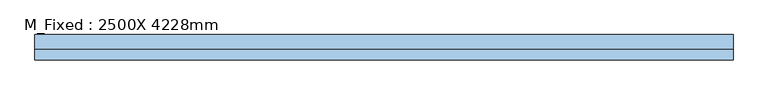
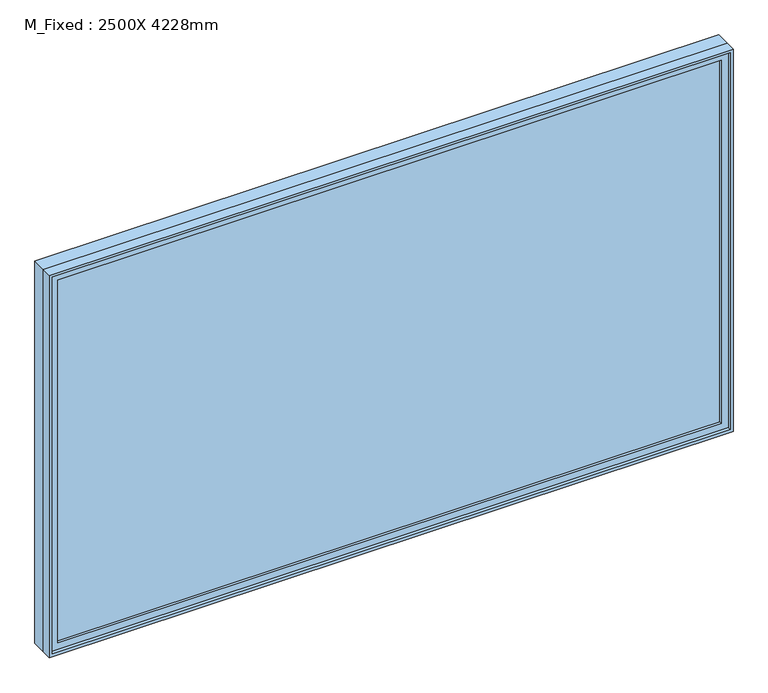
"""IFC4 building model written with IfcOpenShell, lengths in millimetres: window geometry, M_Fixed : 2500X 4228mm."""

import ifcopenshell
import ifcopenshell.guid

model = None  # the IFC model being written
_history = None  # IfcOwnerHistory: only IFC2X3 demands one
_inside = {}  # id of a spatial element -> (the spatial element, [elements in it])
_under = {}  # id of a project, library or spatial element -> (it, [spatial elements below it])
_declared = {}  # id of a project -> (the project, [libraries it declares])
_typed = {}  # id of a type object -> (the type object, [elements of that type])
_made_of = {}  # id of a material, layer set ... -> (it, [elements and type objects made of it])


def new_model(schema):
    """Start an empty IFC model of exactly this schema.

    Asked for "IFC4X3", IfcOpenShell would pick the latest addendum, in which some entities
    have other attributes; the version numbers below select the first issue.
    IFC2X3 requires an IfcOwnerHistory on every rooted entity: one is made here for all.
    """
    global model, _history
    if schema == "IFC4X3":
        model = ifcopenshell.file(schema_version=(4, 3, 0, 0))
    else:
        model = ifcopenshell.file(schema=schema)
    _inside.clear()
    _under.clear()
    _declared.clear()
    _typed.clear()
    _made_of.clear()
    _history = None
    if model.schema == "IFC2X3":
        org = make("IfcOrganization", Name="unknown")
        user = make(
            "IfcPersonAndOrganization",
            ThePerson=make("IfcPerson", FamilyName="unknown"),
            TheOrganization=org,
        )
        app = make(
            "IfcApplication",
            ApplicationDeveloper=org,
            Version="unknown",
            ApplicationFullName="unknown",
            ApplicationIdentifier="unknown",
        )
        _history = make(
            "IfcOwnerHistory",
            OwningUser=user,
            OwningApplication=app,
            ChangeAction="ADDED",
            CreationDate=0,
        )
    return model


def make(cls, **values):
    """One entity of the class cls with the attributes given. An attribute that is None is left unset."""
    return model.create_entity(
        cls, **{name: value for name, value in values.items() if value is not None}
    )


def rooted(cls, **values):
    """An entity with a GlobalId (a new one), such as an element, a storey or a relation."""
    return make(cls, GlobalId=ifcopenshell.guid.new(), OwnerHistory=_history, **values)


def si_unit(unit_type, name, prefix=None):
    """IfcSIUnit, for example si_unit("LENGTHUNIT", "METRE", prefix="MILLI")."""
    return make("IfcSIUnit", UnitType=unit_type, Prefix=prefix, Name=name)


def assignment(units):
    """IfcUnitAssignment: the units of a project."""
    return None if units is None else make("IfcUnitAssignment", Units=units)


def point(xyz):
    """IfcCartesianPoint."""
    return None if xyz is None else make("IfcCartesianPoint", Coordinates=xyz)


def direction(xyz):
    """IfcDirection."""
    return None if xyz is None else make("IfcDirection", DirectionRatios=xyz)


def frame(location, z_axis=None, x_axis=None):
    """IfcAxis2Placement3D, a coordinate frame: its origin and axes. An axis left out is left unset."""
    return make(
        "IfcAxis2Placement3D",
        Location=point(location),
        Axis=direction(z_axis),
        RefDirection=direction(x_axis),
    )


def origin():
    """The frame at (0, 0, 0) with its axes left unset."""
    return frame((0.0, 0.0, 0.0))


def place(relative_to, where):
    """IfcLocalPlacement: puts the frame where relative to a parent placement (None: the world)."""
    return make(
        "IfcLocalPlacement", PlacementRelTo=relative_to, RelativePlacement=where
    )


def context(
    kind, dimensions, precision=None, world=None, true_north=None, identifier=None
):
    """IfcGeometricRepresentationContext, for example the 3D "Model" context."""
    return make(
        "IfcGeometricRepresentationContext",
        ContextIdentifier=identifier,
        ContextType=kind,
        CoordinateSpaceDimension=dimensions,
        Precision=precision,
        WorldCoordinateSystem=world,
        TrueNorth=true_north,
    )


def project(units=None, contexts=None):
    """IfcProject with its units and contexts."""
    return rooted(
        "IfcProject",
        Name="project",
        RepresentationContexts=contexts,
        UnitsInContext=assignment(units),
    )


def spatial(cls, under=None, at=None, **own):
    """A site, building, storey or space (cls), placed at a placement, below another one or the project."""
    s = rooted(cls, ObjectPlacement=at, **own)
    if under is not None:
        _under.setdefault(under.id(), (under, []))[1].append(s)
    return s


def polyline(points):
    """IfcPolyline through the points."""
    return make("IfcPolyline", Points=[point(p) for p in points])


def outline(outer, holes=None, kind="AREA"):
    """IfcArbitraryClosedProfileDef: a profile drawn as a closed curve; with holes, ...WithVoids."""
    if holes is None:
        return make("IfcArbitraryClosedProfileDef", ProfileType=kind, OuterCurve=outer)
    return make(
        "IfcArbitraryProfileDefWithVoids",
        ProfileType=kind,
        OuterCurve=outer,
        InnerCurves=holes,
    )


def extrude(swept, where, along, depth):
    """IfcExtrudedAreaSolid: the profile swept, set in the frame where, extruded along a direction by depth."""
    return make(
        "IfcExtrudedAreaSolid",
        SweptArea=swept,
        Position=where,
        ExtrudedDirection=direction(along),
        Depth=depth,
    )


def shape(context_of_items, identifier, shape_type, items):
    """IfcShapeRepresentation: the items that make up one representation, for example the "Body"."""
    return make(
        "IfcShapeRepresentation",
        ContextOfItems=context_of_items,
        RepresentationIdentifier=identifier,
        RepresentationType=shape_type,
        Items=items,
    )


def source(mapping_origin, context_of_items, identifier, shape_type, items):
    """IfcRepresentationMap: a shape defined once, which mapped items show again and again."""
    return make(
        "IfcRepresentationMap",
        MappingOrigin=mapping_origin,
        MappedRepresentation=shape(context_of_items, identifier, shape_type, items),
    )


def transform(
    local_origin,
    x_axis=None,
    y_axis=None,
    z_axis=None,
    scale=None,
    scale2=None,
    scale3=None,
    uniform=True,
):
    """IfcCartesianTransformationOperator3D, or its non-uniform kind. x_axis, y_axis, z_axis: its Axis1, 2, 3."""
    if uniform:
        return make(
            "IfcCartesianTransformationOperator3D",
            Axis1=direction(x_axis),
            Axis2=direction(y_axis),
            LocalOrigin=point(local_origin),
            Scale=scale,
            Axis3=direction(z_axis),
        )
    return make(
        "IfcCartesianTransformationOperator3DnonUniform",
        Axis1=direction(x_axis),
        Axis2=direction(y_axis),
        LocalOrigin=point(local_origin),
        Scale=scale,
        Axis3=direction(z_axis),
        Scale2=scale2,
        Scale3=scale3,
    )


def mapped(mapping_source, mapping_target):
    """IfcMappedItem: shows the shape of a source again, moved by a transform."""
    return make(
        "IfcMappedItem", MappingSource=mapping_source, MappingTarget=mapping_target
    )


def made_of(thing, what):
    """Note that an element or type object is made of a material, layer set ...; save() writes the relation."""
    if what is not None:
        _made_of.setdefault(what.id(), (what, []))[1].append(thing)
    return thing


def element(
    cls,
    number,
    at=None,
    inside=None,
    cuts=None,
    type_object=None,
    material=None,
    context=None,
    identifier="Body",
    shape_type=None,
    held_by="IfcProductDefinitionShape",
    body=None,
    shapes=None,
    **own,
):
    """One element of the class cls, such as IfcWall. Its Tag is "e" and its number.

    at: its placement. inside: the storey or other place that contains it. cuts: it is an
    opening in that element (IfcRelVoidsElement). A single representation is given by context,
    identifier, shape_type and body (its items); several are given by shapes. held_by: the class
    of the entity that holds the representations. save() writes the other relations.
    """
    e = rooted(cls, Tag="e%d" % number, ObjectPlacement=at, **own)
    if body is not None:
        shapes = [shape(context, identifier, shape_type, body)]
    if shapes is not None:
        e.Representation = make(held_by, Representations=shapes)
    if inside is not None:
        _inside.setdefault(inside.id(), (inside, []))[1].append(e)
    if cuts is not None:
        rooted(
            "IfcRelVoidsElement", RelatingBuildingElement=cuts, RelatedOpeningElement=e
        )
    if type_object is not None:
        _typed.setdefault(type_object.id(), (type_object, []))[1].append(e)
    return made_of(e, material)


def aggregate(whole, parts):
    """IfcRelAggregates: a whole, such as a stair, and the parts it consists of."""
    return rooted("IfcRelAggregates", RelatingObject=whole, RelatedObjects=parts)


def save(model, path):
    """Write the relations noted so far, then the file.

    IfcRelAggregates (storeys below a building ...), IfcRelContainedInSpatialStructure (elements
    in a storey), IfcRelDefinesByType, IfcRelAssociatesMaterial and IfcRelDeclares: one each for
    every whole, place, type object, material and project.
    """
    for whole, parts in _under.values():
        aggregate(whole, parts)
    for where, things in _inside.values():
        rooted(
            "IfcRelContainedInSpatialStructure",
            RelatedElements=things,
            RelatingStructure=where,
        )
    for kind, things in _typed.values():
        rooted("IfcRelDefinesByType", RelatedObjects=things, RelatingType=kind)
    for what, things in _made_of.values():
        rooted("IfcRelAssociatesMaterial", RelatedObjects=things, RelatingMaterial=what)
    for by, libraries in _declared.values():
        rooted("IfcRelDeclares", RelatingContext=by, RelatedDefinitions=libraries)
    model.write(path)


def m_fixed_2500x_4228mm_f14c179f(model_context):
    return source(origin(), model_context, "Body", "SweptSolid", [
        extrude(outline(polyline([(-2050.8, -54.2), (-2050.8, -42.2), (2050.8, -42.2), (2050.8, -54.2), (-2050.8, -54.2)])), frame((0.0, 0.0, 368.0), z_axis=(0.0, 0.0, 1.0), x_axis=(1.0, 0.0, 0.0)), (0.0, 0.0, 1.0), 2374.0),
        extrude(outline(polyline([(2786.0, -2094.8), (324.0, -2094.8), (324.0, 2094.8), (2786.0, 2094.8), (2786.0, -2094.8)]), holes=[polyline([(2742.0, -2050.8), (2742.0, 2050.8), (368.0, 2050.8), (368.0, -2050.8), (2742.0, -2050.8)])]), frame((0.0, -70.2, 0.0), z_axis=(0.0, 1.0, 0.0), x_axis=(0.0, 0.0, 1.0)), (0.0, 0.0, 1.0), 44.0),
        extrude(outline(polyline([(2805.0, -2113.8), (305.0, -2113.8), (305.0, 2113.8), (2805.0, 2113.8), (2805.0, -2113.8)]), holes=[polyline([(2786.0, -2094.8), (2786.0, 2094.8), (324.0, 2094.8), (324.0, -2094.8), (2786.0, -2094.8)])]), frame((0.0, -89.2, 0.0), z_axis=(0.0, 1.0, 0.0), x_axis=(0.0, 0.0, 1.0)), (0.0, 0.0, 1.0), 63.0),
        extrude(outline(polyline([(2805.0, -2113.8), (305.0, -2113.8), (305.0, 2113.8), (2805.0, 2113.8), (2805.0, -2113.8)]), holes=[polyline([(2773.0, -2081.8), (2773.0, 2081.8), (337.0, 2081.8), (337.0, -2081.8), (2773.0, -2081.8)])]), frame((0.0, -26.2, 0.0), z_axis=(0.0, 1.0, 0.0), x_axis=(0.0, 0.0, 1.0)), (0.0, 0.0, 1.0), 89.4),
    ])


if __name__ == "__main__":
    model = new_model("IFC4")
    model_context = context("Model", 3, world=origin())
    ifc_project = project(units=[si_unit("LENGTHUNIT", "METRE", prefix="MILLI")], contexts=[model_context])
    site = spatial("IfcSite", under=ifc_project)
    building = spatial("IfcBuilding", under=site)
    placement = place(None, origin())
    m_fixed_2500x_4228mm_shape = m_fixed_2500x_4228mm_f14c179f(model_context)
    element("IfcWindow", 1, ObjectType="M_Fixed : 2500X 4228mm", at=placement, inside=building, context=model_context, shape_type="MappedRepresentation", body=[
        mapped(m_fixed_2500x_4228mm_shape, transform((0.0, 0.0, 0.0), x_axis=(1.0, 0.0, 0.0), y_axis=(0.0, 1.0, 0.0), z_axis=(0.0, 0.0, 1.0))),
    ])
    save(model, "model.ifc")

# Revit data of these elements
# Type "M_Fixed : 2500X 4228mm"
#   Type Mark = "25"
#   Height = 2500 mm
#   Default Sill Height = 305 mm
#   Width = 4227.6 mm
#   Window Inset = 19 mm
#   Frame Exterior Material = Sash
#   Frame Interior Material = Sash
#   Glass Pane Material = Glass
#   Sash = Sash
#   Wall Closure = (empty or 0)
# Element 1 (IfcWindow, "M_Fixed : 2500X 4228mm")
#   Materials on its faces: "Sash", "Glass"
# Materials
#   "Sash": class "Wood", colour RGB 136 99 55, transparency 0
#   "Glass": class "Glass", colour RGB 0 128 192, transparency 0.9, Description = "Soda Lime Glass", Cost = 0
